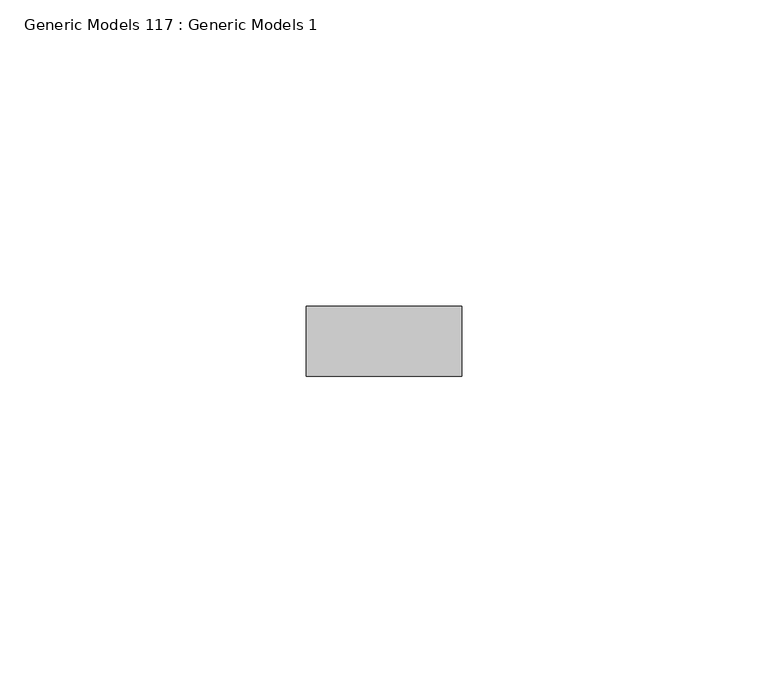
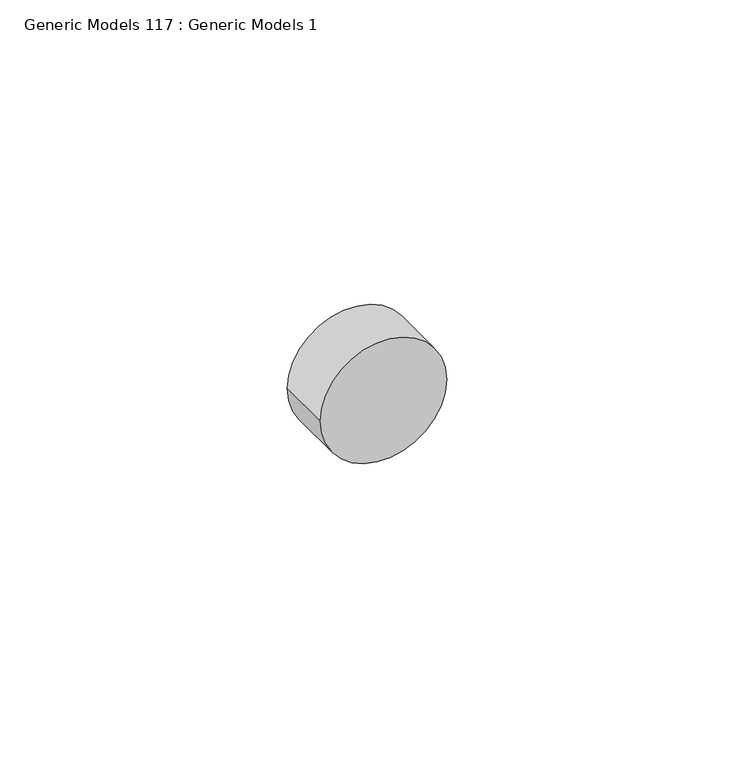
"""IFC4 building model written with IfcOpenShell, lengths in millimetres: proxy geometry, Generic Models 117 : Generic Models 1."""

from ifc_helpers import new_model, si_unit, point, frame, frame_2d, origin, place, context, project, spatial, circle_curve, trimmed, segment, composite_curve, outline, extrude, source, transform, mapped, element, save


def generic_models_117_generic_models_1_df3e69b9(model_context):
    return source(origin(), model_context, "Body", "SweptSolid", [
        extrude(outline(composite_curve([segment(trimmed(circle_curve(frame_2d((38031.9291136, 7128.1828124)), 12.7), [point((38031.9291136, 7115.4828124))], [point((38031.9291136, 7140.8828124))], False, "CARTESIAN"), True, "CONTINUOUS"), segment(trimmed(circle_curve(frame_2d((38031.9291136, 7128.1828124)), 12.7), [point((38031.9291136, 7140.8828124))], [point((38031.9291136, 7115.4828124))], False, "CARTESIAN"), True, "CONTINUOUS")], self_intersect=False)), frame((0.0, 1836.9202358, 0.0), z_axis=(0.0, 1.0, 0.0), x_axis=(0.0, 0.0, 1.0)), (0.0, 0.0, 1.0), 11.4464372),
    ])


if __name__ == "__main__":
    model = new_model("IFC4")
    model_context = context("Model", 3, world=origin())
    ifc_project = project(units=[si_unit("LENGTHUNIT", "METRE", prefix="MILLI")], contexts=[model_context])
    site = spatial("IfcSite", under=ifc_project)
    building = spatial("IfcBuilding", under=site)
    placement = place(None, origin())
    generic_models_117_generic_models_1_shape = generic_models_117_generic_models_1_df3e69b9(model_context)
    element("IfcBuildingElementProxy", 1, Name="Generic Models 117 : Generic Models 1", ObjectType="Generic Models 117 : Generic Models 1", at=placement, inside=building, context=model_context, shape_type="MappedRepresentation", body=[
        mapped(generic_models_117_generic_models_1_shape, transform((0.0, 0.0, 0.0), x_axis=(1.0, 0.0, 0.0), y_axis=(0.0, 1.0, 0.0), z_axis=(0.0, 0.0, 1.0))),
    ])
    save(model, "model.ifc")

# Revit data of these elements
# Element 1 (IfcBuildingElementProxy, "Generic Models 117 : Generic Models 1")
#   Materials on its faces: "S.S. LAG BOLT - SEE STRUCT. DWGS"
# Materials
#   "S.S. LAG BOLT - SEE STRUCT. DWGS": class "Generic", colour RGB 120 120 120, transparency 0, Cost = 0
